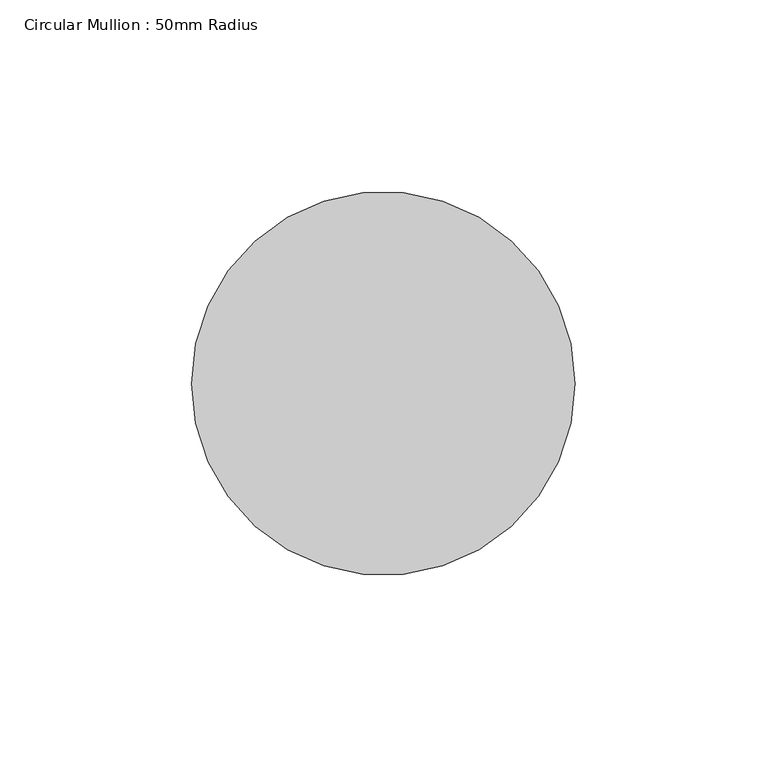
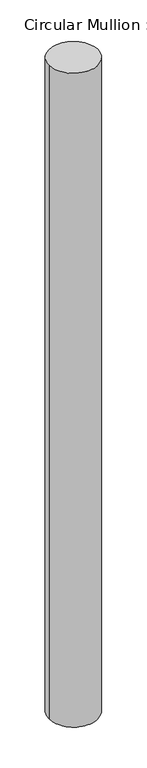
"""IFC4 building model written with IfcOpenShell, lengths in millimetres: member geometry, Circular Mullion : 50mm Radius."""

from ifc_helpers import new_model, si_unit, frame, origin, place, context, project, spatial, ellipse_curve, source, transform, mapped, element, save
from ifc_brep_helpers import plane_surface, cylinder_surface, advanced_brep


def circular_mullion_50mm_radius_c4f49fe3(model_context):
    return source(origin(), model_context, "Body", "AdvancedBrep", [
        advanced_brep(
        [(-100.0, 0.0, 0.4152552), (0.0, 0.0, 0.0), (0.0, 0.0, -1407.9245619), (-100.0, 0.0, -1408.3672765)],
        [
            (0, 1, ellipse_curve(frame((-50.0, 0.0, 0.2076276), z_axis=(-0.004152107286080505, -0.014026987413350105, -0.999892996089677), x_axis=(-0.28380424617451755, -0.9587706469654277, 0.014628614794607739)), 50.0053508, 50.0)),
            (1, 2),
            (2, 3, ellipse_curve(frame((-50.0, 0.0, -1408.1459192), z_axis=(-0.004426608352650427, -0.01495432930035626, 0.9998783791910238), x_axis=(0.2838000973926846, 0.958756631212307, 0.015595731029068905)), 50.0060818, 50.0)),
            (3, 0),
            (1, 0, ellipse_curve(frame((-50.0, 0.0, 0.2076276), z_axis=(-0.004152107286080505, -0.014026987413350105, -0.999892996089677), x_axis=(-0.28380424617451755, -0.9587706469654277, 0.014628614794607739)), 50.0053508, 50.0)),
            (3, 2, ellipse_curve(frame((-50.0, 0.0, -1408.1459192), z_axis=(-0.004426608352650427, -0.01495432930035626, 0.9998783791910238), x_axis=(0.2838000973926846, 0.958756631212307, 0.015595731029068905)), 50.0060818, 50.0)),
        ],
        [
            cylinder_surface(frame((-50.0, 0.0, 0.0), z_axis=(0.0, 0.0, 1.0), x_axis=(1.0, 0.0, 0.0)), 50.0),
            plane_surface(frame((-292.2645666, 86.5127914, 0.0), z_axis=(0.004152107286080505, 0.014026987413350105, 0.999892996089677), x_axis=(0.28380424617451677, 0.9587706469654278, -0.014628614794621025))),
            plane_surface(frame((-292.2645666, 86.5127914, -1407.9245619), z_axis=(0.004426608352650427, 0.01495432930035626, -0.9998783791910238), x_axis=(0.2838000973926845, 0.958756631212307, 0.015595731029074855))),
        ],
        [
            (0, [[1, 2, 3, 4]]),
            (0, [[5, -4, 6, -2]]),
            (1, [[-1, -5]]),
            (2, [[-6, -3]]),
        ],
    ),
    ])


if __name__ == "__main__":
    model = new_model("IFC4")
    model_context = context("Model", 3, world=origin())
    ifc_project = project(units=[si_unit("LENGTHUNIT", "METRE", prefix="MILLI")], contexts=[model_context])
    site = spatial("IfcSite", under=ifc_project)
    building = spatial("IfcBuilding", under=site)
    placement = place(None, origin())
    circular_mullion_50mm_radius_shape = circular_mullion_50mm_radius_c4f49fe3(model_context)
    element("IfcMember", 1, ObjectType="Circular Mullion : 50mm Radius", at=placement, inside=building, context=model_context, shape_type="MappedRepresentation", body=[
        mapped(circular_mullion_50mm_radius_shape, transform((0.0, 0.0, 0.0), x_axis=(1.0, 0.0, 0.0), y_axis=(0.0, 1.0, 0.0), z_axis=(0.0, 0.0, 1.0))),
    ])
    save(model, "model.ifc")

# Revit data of these elements
# Type "Circular Mullion : 50mm Radius"
#   built-in parameter 1007350 = 0.164042 (stored number, unit not read)
# Element 1 (IfcMember, "Circular Mullion : 50mm Radius")
#   Materials on its faces: "Aluminium"
# Materials
#   "Aluminium": class "Metal", colour RGB 247 247 247, transparency 0, Description = "Aluminium 6061", Cost = 0
